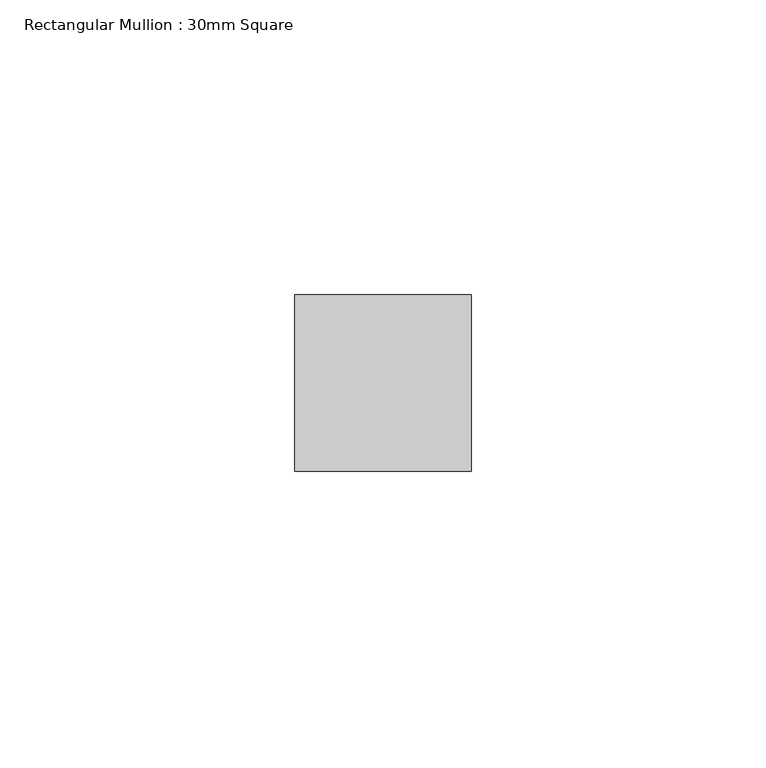
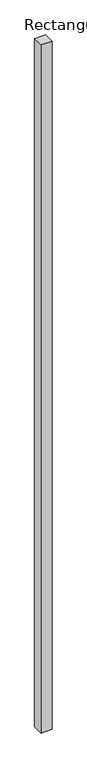
"""IFC4 building model written with IfcOpenShell, lengths in millimetres: member geometry, Rectangular Mullion : 30mm Square."""

from ifc_helpers import new_model, si_unit, frame, origin, place, context, project, spatial, polyline, outline, extrude, source, transform, mapped, element, save


def rectangular_mullion_30mm_square_b082ce79(model_context):
    return source(origin(), model_context, "Body", "SweptSolid", [
        extrude(outline(polyline([(15.0, 15.0), (15.0, -15.0), (-15.0, -15.0), (-15.0, 15.0), (15.0, 15.0)])), frame((0.0, 0.0, -1997.4407133), z_axis=(0.0, 0.0, 1.0), x_axis=(1.0, 0.0, 0.0)), (0.0, 0.0, 1.0), 1997.4407133),
    ])


if __name__ == "__main__":
    model = new_model("IFC4")
    model_context = context("Model", 3, world=origin())
    ifc_project = project(units=[si_unit("LENGTHUNIT", "METRE", prefix="MILLI")], contexts=[model_context])
    site = spatial("IfcSite", under=ifc_project)
    building = spatial("IfcBuilding", under=site)
    placement = place(None, origin())
    rectangular_mullion_30mm_square_shape = rectangular_mullion_30mm_square_b082ce79(model_context)
    element("IfcMember", 1, ObjectType="Rectangular Mullion : 30mm Square", at=placement, inside=building, context=model_context, shape_type="MappedRepresentation", body=[
        mapped(rectangular_mullion_30mm_square_shape, transform((0.0, 0.0, 0.0), x_axis=(1.0, 0.0, 0.0), y_axis=(0.0, 1.0, 0.0), z_axis=(0.0, 0.0, 1.0))),
    ])
    save(model, "model.ifc")

# Revit data of these elements
# Type "Rectangular Mullion : 30mm Square"
#   built-in parameter 1007304 = 0.0984252 (stored number, unit not read)
#   built-in parameter 1007301 = 0.0492126 (stored number, unit not read)
#   built-in parameter 1007300 = 0.0492126 (stored number, unit not read)
# Element 1 (IfcMember, "Rectangular Mullion : 30mm Square")
#   Materials on its faces: "Aluminum"
# Materials
#   "Aluminum": class "Metal", colour RGB 244 244 244, transparency 0, Description = "Aluminum 6061", Cost = 0
